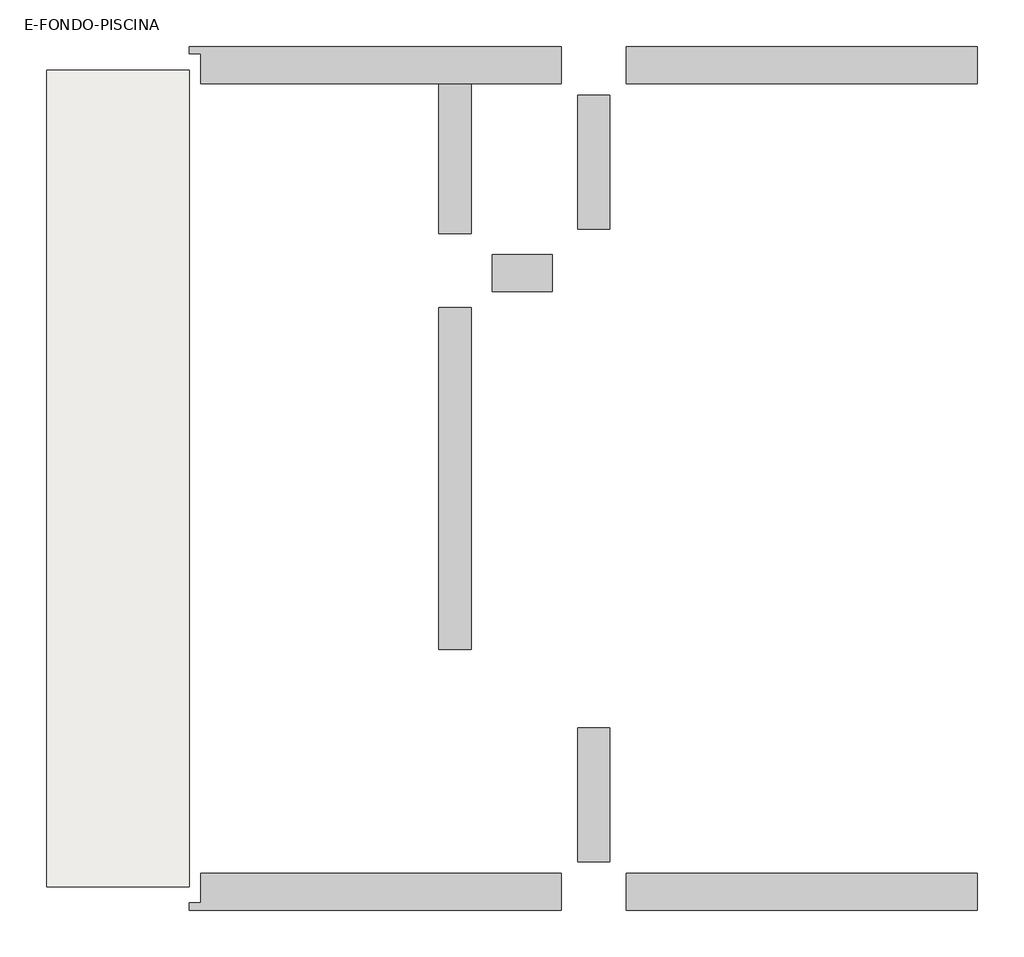
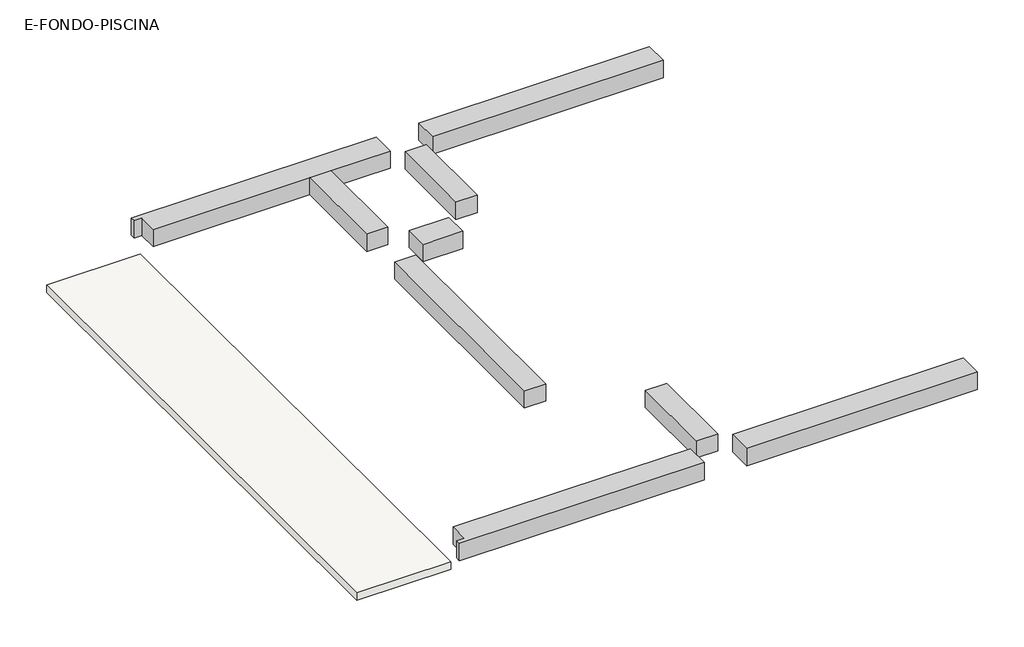
# One storey: 9 beams, 1 slab.
"""IFC4 building model written with IfcOpenShell, lengths in millimetres."""

import ifcopenshell
import ifcopenshell.guid

model = None  # the IFC model being written
_history = None  # IfcOwnerHistory: only IFC2X3 demands one
_inside = {}  # id of a spatial element -> (the spatial element, [elements in it])
_under = {}  # id of a project, library or spatial element -> (it, [spatial elements below it])
_declared = {}  # id of a project -> (the project, [libraries it declares])
_typed = {}  # id of a type object -> (the type object, [elements of that type])
_made_of = {}  # id of a material, layer set ... -> (it, [elements and type objects made of it])


def new_model(schema):
    """Start an empty IFC model of exactly this schema.

    Asked for "IFC4X3", IfcOpenShell would pick the latest addendum, in which some entities
    have other attributes; the version numbers below select the first issue.
    IFC2X3 requires an IfcOwnerHistory on every rooted entity: one is made here for all.
    """
    global model, _history
    if schema == "IFC4X3":
        model = ifcopenshell.file(schema_version=(4, 3, 0, 0))
    else:
        model = ifcopenshell.file(schema=schema)
    _inside.clear()
    _under.clear()
    _declared.clear()
    _typed.clear()
    _made_of.clear()
    _history = None
    if model.schema == "IFC2X3":
        org = make("IfcOrganization", Name="unknown")
        user = make(
            "IfcPersonAndOrganization",
            ThePerson=make("IfcPerson", FamilyName="unknown"),
            TheOrganization=org,
        )
        app = make(
            "IfcApplication",
            ApplicationDeveloper=org,
            Version="unknown",
            ApplicationFullName="unknown",
            ApplicationIdentifier="unknown",
        )
        _history = make(
            "IfcOwnerHistory",
            OwningUser=user,
            OwningApplication=app,
            ChangeAction="ADDED",
            CreationDate=0,
        )
    return model


def make(cls, **values):
    """One entity of the class cls with the attributes given. An attribute that is None is left unset."""
    return model.create_entity(
        cls, **{name: value for name, value in values.items() if value is not None}
    )


def rooted(cls, **values):
    """An entity with a GlobalId (a new one), such as an element, a storey or a relation."""
    return make(cls, GlobalId=ifcopenshell.guid.new(), OwnerHistory=_history, **values)


def si_unit(unit_type, name, prefix=None):
    """IfcSIUnit, for example si_unit("LENGTHUNIT", "METRE", prefix="MILLI")."""
    return make("IfcSIUnit", UnitType=unit_type, Prefix=prefix, Name=name)


def assignment(units):
    """IfcUnitAssignment: the units of a project."""
    return None if units is None else make("IfcUnitAssignment", Units=units)


def point(xyz):
    """IfcCartesianPoint."""
    return None if xyz is None else make("IfcCartesianPoint", Coordinates=xyz)


def direction(xyz):
    """IfcDirection."""
    return None if xyz is None else make("IfcDirection", DirectionRatios=xyz)


def frame(location, z_axis=None, x_axis=None):
    """IfcAxis2Placement3D, a coordinate frame: its origin and axes. An axis left out is left unset."""
    return make(
        "IfcAxis2Placement3D",
        Location=point(location),
        Axis=direction(z_axis),
        RefDirection=direction(x_axis),
    )


def origin():
    """The frame at (0, 0, 0) with its axes left unset."""
    return frame((0.0, 0.0, 0.0))


def place(relative_to, where):
    """IfcLocalPlacement: puts the frame where relative to a parent placement (None: the world)."""
    return make(
        "IfcLocalPlacement", PlacementRelTo=relative_to, RelativePlacement=where
    )


def context(
    kind, dimensions, precision=None, world=None, true_north=None, identifier=None
):
    """IfcGeometricRepresentationContext, for example the 3D "Model" context."""
    return make(
        "IfcGeometricRepresentationContext",
        ContextIdentifier=identifier,
        ContextType=kind,
        CoordinateSpaceDimension=dimensions,
        Precision=precision,
        WorldCoordinateSystem=world,
        TrueNorth=true_north,
    )


def project(units=None, contexts=None):
    """IfcProject with its units and contexts."""
    return rooted(
        "IfcProject",
        Name="project",
        RepresentationContexts=contexts,
        UnitsInContext=assignment(units),
    )


def spatial(cls, under=None, at=None, **own):
    """A site, building, storey or space (cls), placed at a placement, below another one or the project."""
    s = rooted(cls, ObjectPlacement=at, **own)
    if under is not None:
        _under.setdefault(under.id(), (under, []))[1].append(s)
    return s


def polyline(points):
    """IfcPolyline through the points."""
    return make("IfcPolyline", Points=[point(p) for p in points])


def outline(outer, holes=None, kind="AREA"):
    """IfcArbitraryClosedProfileDef: a profile drawn as a closed curve; with holes, ...WithVoids."""
    if holes is None:
        return make("IfcArbitraryClosedProfileDef", ProfileType=kind, OuterCurve=outer)
    return make(
        "IfcArbitraryProfileDefWithVoids",
        ProfileType=kind,
        OuterCurve=outer,
        InnerCurves=holes,
    )


def extrude(swept, where, along, depth):
    """IfcExtrudedAreaSolid: the profile swept, set in the frame where, extruded along a direction by depth."""
    return make(
        "IfcExtrudedAreaSolid",
        SweptArea=swept,
        Position=where,
        ExtrudedDirection=direction(along),
        Depth=depth,
    )


def faces_of(points, faces, orient=None, outer=None):
    """IfcFace entities. A face is a list of loops; a loop is a list of indices into points, from 0.

    orient and outer hold one flag for each loop. By default every Orientation is true, the
    first loop of a face is its IfcFaceOuterBound and the others are IfcFaceBound.
    """
    made = []
    for i, loops in enumerate(faces):
        bounds = []
        for j, loop in enumerate(loops):
            is_outer = j == 0 if outer is None else outer[i][j]
            bounds.append(
                make(
                    "IfcFaceOuterBound" if is_outer else "IfcFaceBound",
                    Bound=make("IfcPolyLoop", Polygon=[points[k] for k in loop]),
                    Orientation=True if orient is None else orient[i][j],
                )
            )
        made.append(make("IfcFace", Bounds=bounds))
    return made


def faceted_brep(points, faces, orient=None, outer=None, voids=None):
    """IfcFacetedBrep: a solid bounded by flat faces; with voids (closed shells), ...WithVoids."""
    shared = [point(p) for p in points]
    hull = make("IfcClosedShell", CfsFaces=faces_of(shared, faces, orient, outer))
    if voids is None:
        return make("IfcFacetedBrep", Outer=hull)
    return make(
        "IfcFacetedBrepWithVoids",
        Outer=hull,
        Voids=[
            make(cls, CfsFaces=faces_of(shared, fs, o, b)) for cls, fs, o, b in voids
        ],
    )


def shape(context_of_items, identifier, shape_type, items):
    """IfcShapeRepresentation: the items that make up one representation, for example the "Body"."""
    return make(
        "IfcShapeRepresentation",
        ContextOfItems=context_of_items,
        RepresentationIdentifier=identifier,
        RepresentationType=shape_type,
        Items=items,
    )


def made_of(thing, what):
    """Note that an element or type object is made of a material, layer set ...; save() writes the relation."""
    if what is not None:
        _made_of.setdefault(what.id(), (what, []))[1].append(thing)
    return thing


def element(
    cls,
    number,
    at=None,
    inside=None,
    cuts=None,
    type_object=None,
    material=None,
    context=None,
    identifier="Body",
    shape_type=None,
    held_by="IfcProductDefinitionShape",
    body=None,
    shapes=None,
    **own,
):
    """One element of the class cls, such as IfcWall. Its Tag is "e" and its number.

    at: its placement. inside: the storey or other place that contains it. cuts: it is an
    opening in that element (IfcRelVoidsElement). A single representation is given by context,
    identifier, shape_type and body (its items); several are given by shapes. held_by: the class
    of the entity that holds the representations. save() writes the other relations.
    """
    e = rooted(cls, Tag="e%d" % number, ObjectPlacement=at, **own)
    if body is not None:
        shapes = [shape(context, identifier, shape_type, body)]
    if shapes is not None:
        e.Representation = make(held_by, Representations=shapes)
    if inside is not None:
        _inside.setdefault(inside.id(), (inside, []))[1].append(e)
    if cuts is not None:
        rooted(
            "IfcRelVoidsElement", RelatingBuildingElement=cuts, RelatedOpeningElement=e
        )
    if type_object is not None:
        _typed.setdefault(type_object.id(), (type_object, []))[1].append(e)
    return made_of(e, material)


def aggregate(whole, parts):
    """IfcRelAggregates: a whole, such as a stair, and the parts it consists of."""
    return rooted("IfcRelAggregates", RelatingObject=whole, RelatedObjects=parts)


def save(model, path):
    """Write the relations noted so far, then the file.

    IfcRelAggregates (storeys below a building ...), IfcRelContainedInSpatialStructure (elements
    in a storey), IfcRelDefinesByType, IfcRelAssociatesMaterial and IfcRelDeclares: one each for
    every whole, place, type object, material and project.
    """
    for whole, parts in _under.values():
        aggregate(whole, parts)
    for where, things in _inside.values():
        rooted(
            "IfcRelContainedInSpatialStructure",
            RelatedElements=things,
            RelatingStructure=where,
        )
    for kind, things in _typed.values():
        rooted("IfcRelDefinesByType", RelatedObjects=things, RelatingType=kind)
    for what, things in _made_of.values():
        rooted("IfcRelAssociatesMaterial", RelatedObjects=things, RelatingMaterial=what)
    for by, libraries in _declared.values():
        rooted("IfcRelDeclares", RelatingContext=by, RelatedDefinitions=libraries)
    model.write(path)


model = new_model("IFC4")

# Units and contexts
model_context = context("Model", 3, world=origin())
ifc_project = project(units=[si_unit("LENGTHUNIT", "METRE", prefix="MILLI")], contexts=[model_context])

# Site, building, storey
site = spatial("IfcSite", under=ifc_project)
building = spatial("IfcBuilding", under=site)
storey = spatial("IfcBuildingStorey", under=building, Name="E-FONDO-PISCINA", Elevation=-1800.0)

# Beams
placement = place(None, origin())
element("IfcBeam", 1, ObjectType="E-VIGA-Hormigon : E-VIGA-Hormigon", at=placement, inside=storey, context=model_context, shape_type="SweptSolid", body=[
    extrude(outline(polyline([(-20300.0, -18350.0), (-20300.0, -17550.0), (-12700.0, -17550.0), (-12700.0, -18350.0), (-20300.0, -18350.0)])), frame((0.0, 0.0, -1500.0), z_axis=(0.0, 0.0, 1.0), x_axis=(1.0, 0.0, 0.0)), (0.0, 0.0, 1.0), 600.0),
])
element("IfcBeam", 2, ObjectType="E-VIGA-Hormigon : E-VIGA-Hormigon", at=placement, inside=storey, context=model_context, shape_type="SweptSolid", body=[
    extrude(outline(polyline([(-21900.0, -4150.0), (-21900.0, -4950.0), (-23200.0, -4950.0), (-23200.0, -4150.0), (-21900.0, -4150.0)])), frame((0.0, 0.0, -1500.0), z_axis=(0.0, 0.0, 1.0), x_axis=(1.0, 0.0, 0.0)), (0.0, 0.0, 1.0), 600.0),
])
element("IfcBeam", 3, ObjectType="E-VIGA-Hormigon : E-VIGA-Hormigon", at=placement, inside=storey, context=model_context, shape_type="SweptSolid", body=[
    extrude(outline(polyline([(-20650.0, -17300.0), (-21350.0, -17300.0), (-21350.0, -14400.0), (-20650.0, -14400.0), (-20650.0, -17300.0)])), frame((0.0, 0.0, -1500.0), z_axis=(0.0, 0.0, 1.0), x_axis=(1.0, 0.0, 0.0)), (0.0, 0.0, 1.0), 600.0),
])
element("IfcBeam", 4, ObjectType="E-VIGA-Hormigon : E-VIGA-Hormigon", at=placement, inside=storey, context=model_context, shape_type="SweptSolid", body=[
    extrude(outline(polyline([(-20650.0, -3600.0), (-21350.0, -3600.0), (-21350.0, -700.0), (-20650.0, -700.0), (-20650.0, -3600.0)])), frame((0.0, 0.0, -1500.0), z_axis=(0.0, 0.0, 1.0), x_axis=(1.0, 0.0, 0.0)), (0.0, 0.0, 1.0), 600.0),
])
element("IfcBeam", 5, ObjectType="E-VIGA-Hormigon : E-VIGA-Hormigon", at=placement, inside=storey, context=model_context, shape_type="Brep", body=[
    faceted_brep([(-23650.0, -5300.0, -1500.0), (-23650.0, -5300.0, -900.0), (-23650.0, -8650.0, -900.0), (-23650.0, -9350.0, -900.0), (-23650.0, -12700.0, -900.0), (-23650.0, -12700.0, -1500.0), (-23650.0, -9350.0, -1500.0), (-23650.0, -8650.0, -1500.0), (-24350.0, -5300.0, -1500.0), (-24350.0, -12700.0, -1500.0), (-24350.0, -5300.0, -900.0), (-24350.0, -12700.0, -900.0)], [[[0, 1, 2, 3, 4, 5, 6, 7]], [[8, 0, 7, 6, 5, 9]], [[10, 8, 9, 11]], [[1, 10, 11, 4, 3, 2]], [[1, 0, 8, 10]], [[5, 4, 11, 9]]]),
])
element("IfcBeam", 6, ObjectType="E-VIGA-Hormigon : E-VIGA-Hormigon", at=placement, inside=storey, context=model_context, shape_type="SweptSolid", body=[
    extrude(outline(polyline([(-23650.0, -3700.0), (-24350.0, -3700.0), (-24350.0, -450.0), (-23650.0, -450.0), (-23650.0, -3700.0)])), frame((0.0, 0.0, -1500.0), z_axis=(0.0, 0.0, 1.0), x_axis=(1.0, 0.0, 0.0)), (0.0, 0.0, 1.0), 600.0),
])
element("IfcBeam", 7, ObjectType="E-VIGA-Hormigon : E-VIGA-Hormigon", at=placement, inside=storey, context=model_context, shape_type="SweptSolid", body=[
    extrude(outline(polyline([(-12700.0, 350.0), (-12700.0, -450.0), (-20300.0, -450.0), (-20300.0, 350.0), (-12700.0, 350.0)])), frame((0.0, 0.0, -1500.0), z_axis=(0.0, 0.0, 1.0), x_axis=(1.0, 0.0, 0.0)), (0.0, 0.0, 1.0), 600.0),
])
element("IfcBeam", 8, ObjectType="E-VIGA-Hormigon : E-VIGA-Hormigon", at=placement, inside=storey, context=model_context, shape_type="Brep", body=[
    faceted_brep([(-29750.0, 350.0, -1500.0), (-29750.0, 350.0, -900.0), (-21700.0, 350.0, -900.0), (-21700.0, 350.0, -1500.0), (-29750.0, 190.0, -1500.0), (-21700.0, -450.0, -1500.0), (-23650.0, -450.0, -1500.0), (-24350.0, -450.0, -1500.0), (-29500.0, -450.0, -1500.0), (-29500.0, 190.0, -1500.0), (-29500.0, -450.0, -900.0), (-21700.0, -450.0, -900.0), (-23650.0, -450.0, -900.0), (-24350.0, -450.0, -900.0), (-29750.0, 190.0, -900.0), (-29500.0, 190.0, -900.0)], [[[0, 1, 2, 3]], [[4, 0, 3, 5, 6, 7, 8, 9]], [[10, 8, 7, 6, 5, 11, 12, 13]], [[1, 14, 15, 10, 13, 12, 11, 2]], [[9, 15, 14, 4]], [[15, 9, 8, 10]], [[1, 0, 4, 14]], [[3, 2, 11, 5]]]),
])
element("IfcBeam", 9, ObjectType="E-VIGA-Hormigon : E-VIGA-Hormigon", at=placement, inside=storey, context=model_context, shape_type="Brep", body=[
    faceted_brep([(-29750.0, -18350.0, -900.0), (-29750.0, -18350.0, -1500.0), (-21700.0, -18350.0, -1500.0), (-21700.0, -18350.0, -900.0), (-29500.0, -18190.0, -1500.0), (-29500.0, -17550.0, -1500.0), (-24350.0, -17550.0, -1500.0), (-23650.0, -17550.0, -1500.0), (-21700.0, -17550.0, -1500.0), (-29750.0, -18190.0, -1500.0), (-29500.0, -17550.0, -900.0), (-24350.0, -17550.0, -900.0), (-23650.0, -17550.0, -900.0), (-21700.0, -17550.0, -900.0), (-29500.0, -18190.0, -900.0), (-29750.0, -18190.0, -900.0)], [[[0, 1, 2, 3]], [[4, 5, 6, 7, 8, 2, 1, 9]], [[5, 10, 11, 12, 13, 8, 7, 6]], [[10, 14, 15, 0, 3, 13, 12, 11]], [[1, 0, 15, 9]], [[4, 14, 10, 5]], [[3, 2, 8, 13]], [[14, 4, 9, 15]]]),
])

# Slab
element("IfcSlab", 10, ObjectType="LOSA VASO PISCINA_PABLO", at=placement, inside=storey, context=model_context, shape_type="SweptSolid", body=[
    extrude(outline(polyline([(-32840.0, -160.0), (-29750.0, -160.0), (-29750.0, -17840.0), (-32840.0, -17840.0), (-32840.0, -160.0)])), frame((0.0, 0.0, -2100.0), z_axis=(0.0, 0.0, 1.0), x_axis=(1.0, 0.0, 0.0)), (0.0, 0.0, 1.0), 250.0),
])

save(model, "model.ifc")

# Revit data of these elements
# Project information
#   Fecha de emisión de proyecto = "Fecha de emisión"
#   Estado de proyecto = "Estado de proyecto"
#   Nombre de cliente = "Propietario"
#   Dirección de proyecto = "Introduzca dirección aquí"
#   Nombre de proyecto = "Nombre de proyecto"
#   Número de proyecto = "0001"
# Grids (mm)
#   "E-6": line (0, 9189.325) -> (0, -29213.653)
#   "E-B": line (7688.401, -13500) -> (-37134.551, -13500)
#   "E-A": line (7688.401, -18000) -> (-37134.551, -18000)
#   "E-BC": line (7688.401, -9000) -> (-37134.551, -9000)
#   "E-C": line (7688.401, -4500) -> (-37134.551, -4500)
#   "E-D": line (7688.401, 0) -> (-37134.551, 0)
#   "E-56": line (-6000, 9189.325) -> (-6000, -29213.653)
#   "E-5": line (-9000, 9189.325) -> (-9000, -29213.653)
#   "E-4": line (-12000, 9189.325) -> (-12000, -29213.653)
#   "E-3": line (-21000, 9189.325) -> (-21000, -29213.653)
#   "E-2": line (-24000, 9189.325) -> (-24000, -29213.653)
#   "E-12": line (-27000, 9189.325) -> (-27000, -29213.653)
#   "E-1": line (-33000, 9189.325) -> (-33000, -29213.653)
#   "E-10": line (-29500, 9189.325) -> (-29500, -29213.653)
# Type "E-VIGA-Hormigon : E-VIGA-Hormigon"
#   Numeration [instance default] = ""
#   Length [instance default] = 3.000 m
#   AnchoViga [instance default] = 0.200 m
#   AltoViga [instance default] = 0.300 m
# Type "LOSA VASO PISCINA_PABLO"
#   Layers, outside or top first: 0.250 m "Hormigón - Hormigón moldeado in situ" (function 1)
# Elements 1, 2, 7, 8, 9 (IfcBeam, "E-VIGA-Hormigon : E-VIGA-Hormigon")
#   Comments = ""
#   Numeration = ""
#   AnchoViga = 0.800 m
#   AltoViga = 0.600 m
#   Phase Created = Nueva construcción
#   Materials on its faces: "Concrete, Cast-in-Place, Gray"
# Elements 3, 4, 5, 6 (IfcBeam, "E-VIGA-Hormigon : E-VIGA-Hormigon")
#   Comments = ""
#   Numeration = ""
#   AnchoViga = 0.700 m
#   AltoViga = 0.600 m
#   Phase Created = Nueva construcción
#   Materials on its faces: "Concrete, Cast-in-Place, Gray"
# Element 10 (IfcSlab, "LOSA VASO PISCINA_PABLO")
#   built-in parameter 1001955 = 1.5708 (stored number, unit not read)
#   Height Offset From Level = -0.050 m
#   built-in parameter 1001954 = 1
#   Phase Created = Nueva construcción
#   Materials on its faces: "Hormigón - Hormigón moldeado in situ"
# Materials
#   "Hormigón - Hormigón moldeado in situ": class "Hormigón", colour RGB 192 192 192, transparency 0, Cost = 0
#   "Concrete, Cast-in-Place, Gray": class "Concrete", colour RGB 129 132 118, transparency 0, Description = "Cast-in-place concrete", Cost = 0
